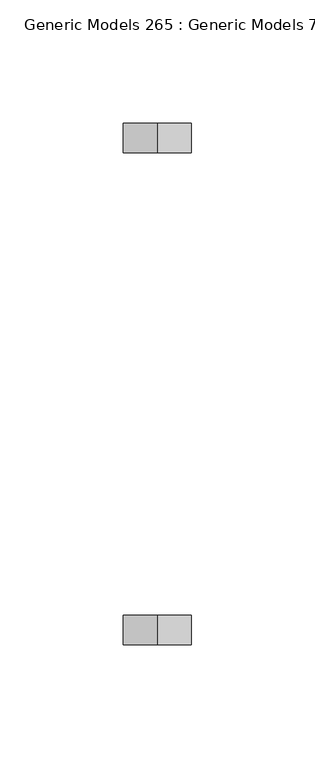
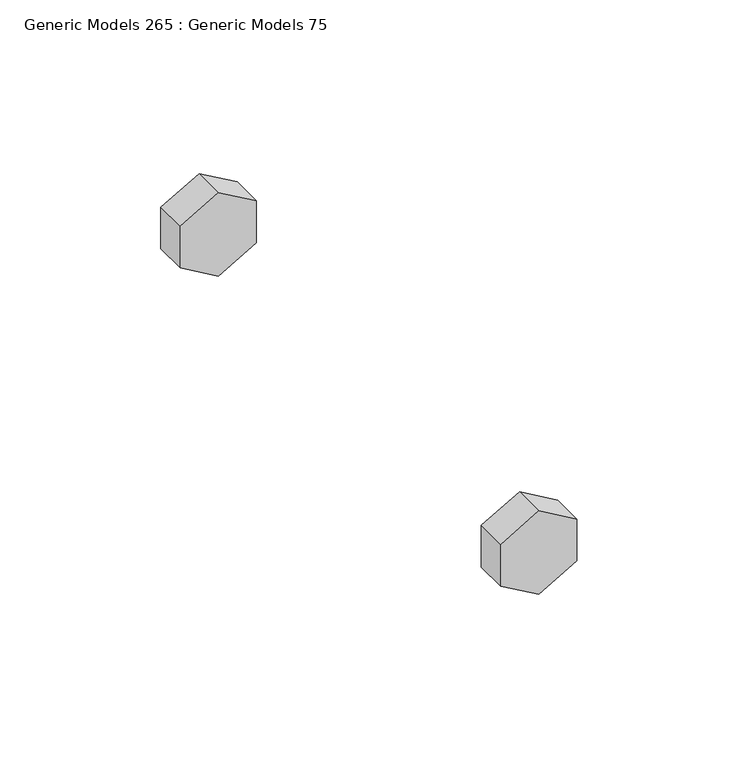
"""IFC4 building model written with IfcOpenShell, lengths in millimetres: proxy geometry, Generic Models 265 : Generic Models 75."""

import ifcopenshell
import ifcopenshell.guid

model = None  # the IFC model being written
_history = None  # IfcOwnerHistory: only IFC2X3 demands one
_inside = {}  # id of a spatial element -> (the spatial element, [elements in it])
_under = {}  # id of a project, library or spatial element -> (it, [spatial elements below it])
_declared = {}  # id of a project -> (the project, [libraries it declares])
_typed = {}  # id of a type object -> (the type object, [elements of that type])
_made_of = {}  # id of a material, layer set ... -> (it, [elements and type objects made of it])


def new_model(schema):
    """Start an empty IFC model of exactly this schema.

    Asked for "IFC4X3", IfcOpenShell would pick the latest addendum, in which some entities
    have other attributes; the version numbers below select the first issue.
    IFC2X3 requires an IfcOwnerHistory on every rooted entity: one is made here for all.
    """
    global model, _history
    if schema == "IFC4X3":
        model = ifcopenshell.file(schema_version=(4, 3, 0, 0))
    else:
        model = ifcopenshell.file(schema=schema)
    _inside.clear()
    _under.clear()
    _declared.clear()
    _typed.clear()
    _made_of.clear()
    _history = None
    if model.schema == "IFC2X3":
        org = make("IfcOrganization", Name="unknown")
        user = make(
            "IfcPersonAndOrganization",
            ThePerson=make("IfcPerson", FamilyName="unknown"),
            TheOrganization=org,
        )
        app = make(
            "IfcApplication",
            ApplicationDeveloper=org,
            Version="unknown",
            ApplicationFullName="unknown",
            ApplicationIdentifier="unknown",
        )
        _history = make(
            "IfcOwnerHistory",
            OwningUser=user,
            OwningApplication=app,
            ChangeAction="ADDED",
            CreationDate=0,
        )
    return model


def make(cls, **values):
    """One entity of the class cls with the attributes given. An attribute that is None is left unset."""
    return model.create_entity(
        cls, **{name: value for name, value in values.items() if value is not None}
    )


def rooted(cls, **values):
    """An entity with a GlobalId (a new one), such as an element, a storey or a relation."""
    return make(cls, GlobalId=ifcopenshell.guid.new(), OwnerHistory=_history, **values)


def si_unit(unit_type, name, prefix=None):
    """IfcSIUnit, for example si_unit("LENGTHUNIT", "METRE", prefix="MILLI")."""
    return make("IfcSIUnit", UnitType=unit_type, Prefix=prefix, Name=name)


def assignment(units):
    """IfcUnitAssignment: the units of a project."""
    return None if units is None else make("IfcUnitAssignment", Units=units)


def point(xyz):
    """IfcCartesianPoint."""
    return None if xyz is None else make("IfcCartesianPoint", Coordinates=xyz)


def direction(xyz):
    """IfcDirection."""
    return None if xyz is None else make("IfcDirection", DirectionRatios=xyz)


def frame(location, z_axis=None, x_axis=None):
    """IfcAxis2Placement3D, a coordinate frame: its origin and axes. An axis left out is left unset."""
    return make(
        "IfcAxis2Placement3D",
        Location=point(location),
        Axis=direction(z_axis),
        RefDirection=direction(x_axis),
    )


def origin():
    """The frame at (0, 0, 0) with its axes left unset."""
    return frame((0.0, 0.0, 0.0))


def place(relative_to, where):
    """IfcLocalPlacement: puts the frame where relative to a parent placement (None: the world)."""
    return make(
        "IfcLocalPlacement", PlacementRelTo=relative_to, RelativePlacement=where
    )


def context(
    kind, dimensions, precision=None, world=None, true_north=None, identifier=None
):
    """IfcGeometricRepresentationContext, for example the 3D "Model" context."""
    return make(
        "IfcGeometricRepresentationContext",
        ContextIdentifier=identifier,
        ContextType=kind,
        CoordinateSpaceDimension=dimensions,
        Precision=precision,
        WorldCoordinateSystem=world,
        TrueNorth=true_north,
    )


def project(units=None, contexts=None):
    """IfcProject with its units and contexts."""
    return rooted(
        "IfcProject",
        Name="project",
        RepresentationContexts=contexts,
        UnitsInContext=assignment(units),
    )


def spatial(cls, under=None, at=None, **own):
    """A site, building, storey or space (cls), placed at a placement, below another one or the project."""
    s = rooted(cls, ObjectPlacement=at, **own)
    if under is not None:
        _under.setdefault(under.id(), (under, []))[1].append(s)
    return s


def polyline(points):
    """IfcPolyline through the points."""
    return make("IfcPolyline", Points=[point(p) for p in points])


def outline(outer, holes=None, kind="AREA"):
    """IfcArbitraryClosedProfileDef: a profile drawn as a closed curve; with holes, ...WithVoids."""
    if holes is None:
        return make("IfcArbitraryClosedProfileDef", ProfileType=kind, OuterCurve=outer)
    return make(
        "IfcArbitraryProfileDefWithVoids",
        ProfileType=kind,
        OuterCurve=outer,
        InnerCurves=holes,
    )


def extrude(swept, where, along, depth):
    """IfcExtrudedAreaSolid: the profile swept, set in the frame where, extruded along a direction by depth."""
    return make(
        "IfcExtrudedAreaSolid",
        SweptArea=swept,
        Position=where,
        ExtrudedDirection=direction(along),
        Depth=depth,
    )


def shape(context_of_items, identifier, shape_type, items):
    """IfcShapeRepresentation: the items that make up one representation, for example the "Body"."""
    return make(
        "IfcShapeRepresentation",
        ContextOfItems=context_of_items,
        RepresentationIdentifier=identifier,
        RepresentationType=shape_type,
        Items=items,
    )


def source(mapping_origin, context_of_items, identifier, shape_type, items):
    """IfcRepresentationMap: a shape defined once, which mapped items show again and again."""
    return make(
        "IfcRepresentationMap",
        MappingOrigin=mapping_origin,
        MappedRepresentation=shape(context_of_items, identifier, shape_type, items),
    )


def transform(
    local_origin,
    x_axis=None,
    y_axis=None,
    z_axis=None,
    scale=None,
    scale2=None,
    scale3=None,
    uniform=True,
):
    """IfcCartesianTransformationOperator3D, or its non-uniform kind. x_axis, y_axis, z_axis: its Axis1, 2, 3."""
    if uniform:
        return make(
            "IfcCartesianTransformationOperator3D",
            Axis1=direction(x_axis),
            Axis2=direction(y_axis),
            LocalOrigin=point(local_origin),
            Scale=scale,
            Axis3=direction(z_axis),
        )
    return make(
        "IfcCartesianTransformationOperator3DnonUniform",
        Axis1=direction(x_axis),
        Axis2=direction(y_axis),
        LocalOrigin=point(local_origin),
        Scale=scale,
        Axis3=direction(z_axis),
        Scale2=scale2,
        Scale3=scale3,
    )


def mapped(mapping_source, mapping_target):
    """IfcMappedItem: shows the shape of a source again, moved by a transform."""
    return make(
        "IfcMappedItem", MappingSource=mapping_source, MappingTarget=mapping_target
    )


def made_of(thing, what):
    """Note that an element or type object is made of a material, layer set ...; save() writes the relation."""
    if what is not None:
        _made_of.setdefault(what.id(), (what, []))[1].append(thing)
    return thing


def element(
    cls,
    number,
    at=None,
    inside=None,
    cuts=None,
    type_object=None,
    material=None,
    context=None,
    identifier="Body",
    shape_type=None,
    held_by="IfcProductDefinitionShape",
    body=None,
    shapes=None,
    **own,
):
    """One element of the class cls, such as IfcWall. Its Tag is "e" and its number.

    at: its placement. inside: the storey or other place that contains it. cuts: it is an
    opening in that element (IfcRelVoidsElement). A single representation is given by context,
    identifier, shape_type and body (its items); several are given by shapes. held_by: the class
    of the entity that holds the representations. save() writes the other relations.
    """
    e = rooted(cls, Tag="e%d" % number, ObjectPlacement=at, **own)
    if body is not None:
        shapes = [shape(context, identifier, shape_type, body)]
    if shapes is not None:
        e.Representation = make(held_by, Representations=shapes)
    if inside is not None:
        _inside.setdefault(inside.id(), (inside, []))[1].append(e)
    if cuts is not None:
        rooted(
            "IfcRelVoidsElement", RelatingBuildingElement=cuts, RelatedOpeningElement=e
        )
    if type_object is not None:
        _typed.setdefault(type_object.id(), (type_object, []))[1].append(e)
    return made_of(e, material)


def aggregate(whole, parts):
    """IfcRelAggregates: a whole, such as a stair, and the parts it consists of."""
    return rooted("IfcRelAggregates", RelatingObject=whole, RelatedObjects=parts)


def save(model, path):
    """Write the relations noted so far, then the file.

    IfcRelAggregates (storeys below a building ...), IfcRelContainedInSpatialStructure (elements
    in a storey), IfcRelDefinesByType, IfcRelAssociatesMaterial and IfcRelDeclares: one each for
    every whole, place, type object, material and project.
    """
    for whole, parts in _under.values():
        aggregate(whole, parts)
    for where, things in _inside.values():
        rooted(
            "IfcRelContainedInSpatialStructure",
            RelatedElements=things,
            RelatingStructure=where,
        )
    for kind, things in _typed.values():
        rooted("IfcRelDefinesByType", RelatedObjects=things, RelatingType=kind)
    for what, things in _made_of.values():
        rooted("IfcRelAssociatesMaterial", RelatedObjects=things, RelatingMaterial=what)
    for by, libraries in _declared.values():
        rooted("IfcRelDeclares", RelatingContext=by, RelatedDefinitions=libraries)
    model.write(path)


def generic_models_265_generic_models_75_6174bfeb(model_context):
    return source(origin(), model_context, "Body", "SweptSolid", [
        extrude(outline(polyline([(268841.3462802, 31975.9942029), (268825.5097067, 31975.9942029), (268817.59142, 31989.7090778), (268825.5097067, 32003.4239528), (268841.3462802, 32003.4239528), (268849.264567, 31989.7090778), (268841.3462802, 31975.9942029)])), frame((0.0, 30868.0031612, 0.0), z_axis=(0.0, 1.0, 0.0), x_axis=(0.0, 0.0, 1.0)), (0.0, 0.0, 1.0), 11.90625),
        extrude(outline(polyline([(268841.3462802, 31975.9942029), (268825.5097067, 31975.9942029), (268817.59142, 31989.7090778), (268825.5097067, 32003.4239528), (268841.3462802, 32003.4239528), (268849.264567, 31989.7090778), (268841.3462802, 31975.9942029)])), frame((0.0, 30668.7719112, 0.0), z_axis=(0.0, 1.0, 0.0), x_axis=(0.0, 0.0, 1.0)), (0.0, 0.0, 1.0), 11.90625),
    ])


if __name__ == "__main__":
    model = new_model("IFC4")
    model_context = context("Model", 3, world=origin())
    ifc_project = project(units=[si_unit("LENGTHUNIT", "METRE", prefix="MILLI")], contexts=[model_context])
    site = spatial("IfcSite", under=ifc_project)
    building = spatial("IfcBuilding", under=site)
    placement = place(None, origin())
    generic_models_265_generic_models_75_shape = generic_models_265_generic_models_75_6174bfeb(model_context)
    element("IfcBuildingElementProxy", 1, Name="Generic Models 265 : Generic Models 75", ObjectType="Generic Models 265 : Generic Models 75", at=placement, inside=building, context=model_context, shape_type="MappedRepresentation", body=[
        mapped(generic_models_265_generic_models_75_shape, transform((0.0, 0.0, 0.0), x_axis=(1.0, 0.0, 0.0), y_axis=(0.0, 1.0, 0.0), z_axis=(0.0, 0.0, 1.0))),
    ])
    save(model, "model.ifc")

# Revit data of these elements
# Element 1 (IfcBuildingElementProxy, "Generic Models 265 : Generic Models 75")
#   Materials on its faces: "3/4\" GALV. THRU BOLTS"
# Materials
#   "3/4\" GALV. THRU BOLTS": class "Generic", colour RGB 105 69 171, transparency 0, Cost = 0
